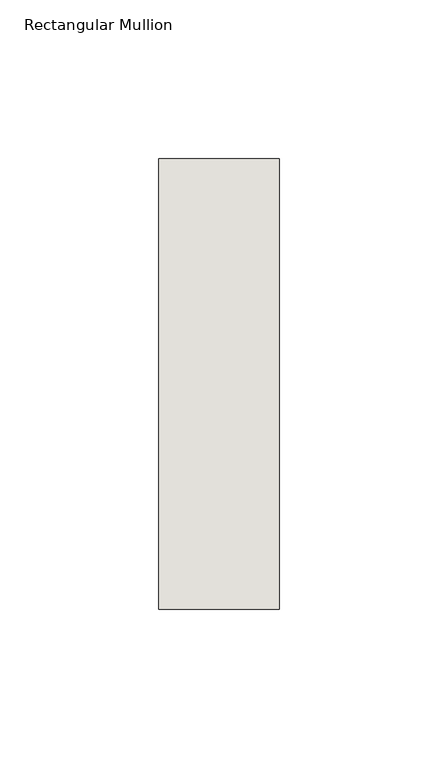
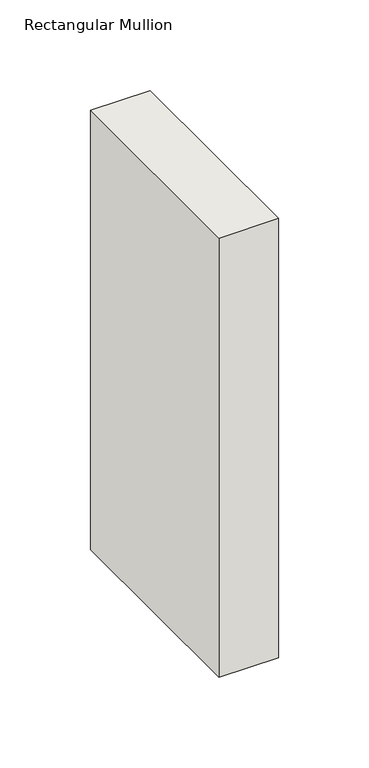
"""IFC4 building model written with IfcOpenShell, lengths in millimetres: wall geometry, Rectangular Mullion : NLRS_21_CWM_hsb-regel 38x142_gen_rsf."""

from ifc_helpers import new_model, si_unit, frame, origin, place, context, project, spatial, polyline, outline, extrude, source, transform, mapped, element, save


def rectangular_mullion_67144ce8(model_context):
    return source(origin(), model_context, "Body", "SweptSolid", [
        extrude(outline(polyline([(19.0, -71.0), (-19.0, -71.0), (-19.0, 71.0), (19.0, 71.0), (19.0, -71.0)])), frame((0.0, 0.0, -296.0), z_axis=(0.0, 0.0, 1.0), x_axis=(1.0, 0.0, 0.0)), (0.0, 0.0, 1.0), 296.0),
    ])


if __name__ == "__main__":
    model = new_model("IFC4")
    model_context = context("Model", 3, world=origin())
    ifc_project = project(units=[si_unit("LENGTHUNIT", "METRE", prefix="MILLI")], contexts=[model_context])
    site = spatial("IfcSite", under=ifc_project)
    building = spatial("IfcBuilding", under=site)
    placement = place(None, origin())
    rectangular_mullion_shape = rectangular_mullion_67144ce8(model_context)
    element("IfcWall", 1, ObjectType="Rectangular Mullion : NLRS_21_CWM_hsb-regel 38x142_gen_rsf", at=placement, inside=building, context=model_context, shape_type="MappedRepresentation", body=[
        mapped(rectangular_mullion_shape, transform((0.0, 0.0, 0.0), x_axis=(1.0, 0.0, 0.0), y_axis=(0.0, 1.0, 0.0), z_axis=(0.0, 0.0, 1.0))),
    ])
    save(model, "model.ifc")

# Revit data of these elements
# Type "Rectangular Mullion : NLRS_21_CWM_hsb-regel 38x142_gen_rsf"
#   Type IfcGUID = "07M7mRoiH1CR8m_RSKIwpF"
#   Assembly Code = "21.10"
#   IfcExportAs = "IfcWall"
#   built-in parameter 1007322 = 0.465879 (stored number, unit not read)
#   built-in parameter 1007321 = 0.062336 (stored number, unit not read)
#   built-in parameter 1007320 = 0.062336 (stored number, unit not read)
# Element 1 (IfcWall, "Rectangular Mullion : NLRS_21_CWM_hsb-regel 38x142_gen_rsf")
#   Materials on its faces: "NLRS_i2_hout naaldhout vuren_gen_rsf"
# Materials
#   "NLRS_i2_hout naaldhout vuren_gen_rsf": class "I - Hout", colour RGB 234 199 147, transparency 0, Keynote = "i2", Manufacturer = "Revit Standards Foundation", URL = "www.revitstandards.org", Description = "hout vuren", Cost = 0
